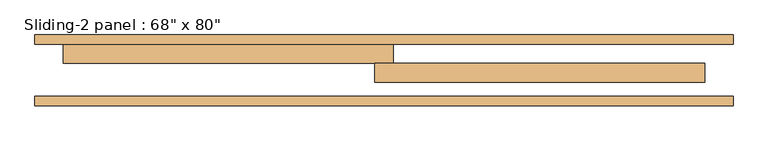
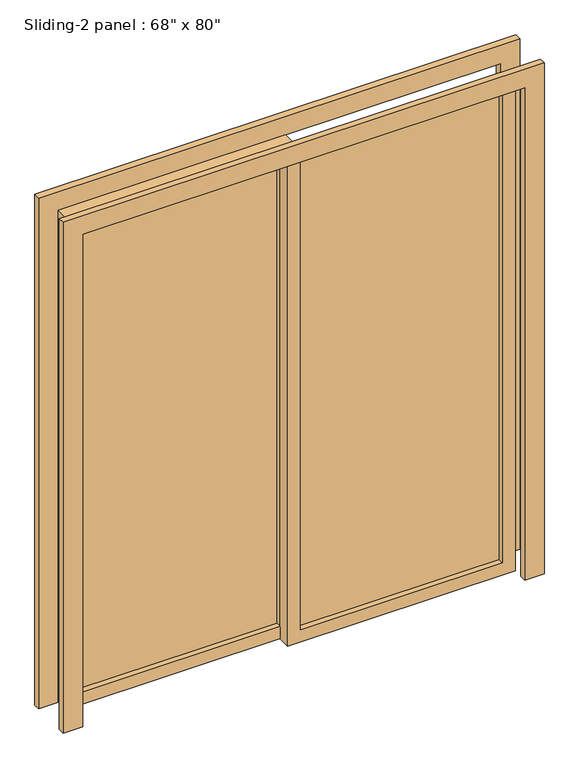
"""IFC4 building model written with IfcOpenShell, lengths in millimetres: door geometry."""

from ifc_helpers import new_model, si_unit, frame, origin, place, context, project, spatial, polyline, outline, extrude, source, transform, mapped, element, save


def door_e1f4216b(model_context):
    return source(origin(), model_context, "Body", "SweptSolid", [
        extrude(outline(polyline([(25.4, 123.825), (812.8, 123.825), (812.8, 117.475), (25.4, 117.475), (25.4, 123.825)])), frame((0.0, 0.0, 50.8), z_axis=(0.0, 0.0, 1.0), x_axis=(1.0, 0.0, 0.0)), (0.0, 0.0, 1.0), 1930.4),
        extrude(outline(polyline([(2032.0, -25.4), (0.0, -25.4), (0.0, 863.6), (2032.0, 863.6), (2032.0, -25.4)]), holes=[polyline([(1981.2, 25.4), (1981.2, 812.8), (50.8, 812.8), (50.8, 25.4), (1981.2, 25.4)])]), frame((0.0, 95.25, 0.0), z_axis=(0.0, 1.0, 0.0), x_axis=(0.0, 0.0, 1.0)), (0.0, 0.0, 1.0), 50.8),
        extrude(outline(polyline([(-812.8, 174.625), (-25.4, 174.625), (-25.4, 168.275), (-812.8, 168.275), (-812.8, 174.625)])), frame((0.0, 0.0, 50.8), z_axis=(0.0, 0.0, 1.0), x_axis=(1.0, 0.0, 0.0)), (0.0, 0.0, 1.0), 1930.4),
        extrude(outline(polyline([(2032.0, 25.4), (2032.0, -863.6), (0.0, -863.6), (0.0, 25.4), (2032.0, 25.4)]), holes=[polyline([(1981.2, -25.4), (50.8, -25.4), (50.8, -812.8), (1981.2, -812.8), (1981.2, -25.4)])]), frame((0.0, 146.05, 0.0), z_axis=(0.0, 1.0, 0.0), x_axis=(0.0, 0.0, 1.0)), (0.0, 0.0, 1.0), 50.8),
        extrude(outline(polyline([(0.0, -939.8), (0.0, -863.6), (2032.0, -863.6), (2032.0, 863.6), (0.0, 863.6), (0.0, 939.8), (2108.2, 939.8), (2108.2, -939.8), (0.0, -939.8)])), frame((0.0, 31.75, 0.0), z_axis=(0.0, 1.0, 0.0), x_axis=(0.0, 0.0, 1.0)), (0.0, 0.0, 1.0), 25.4),
        extrude(outline(polyline([(0.0, 939.8), (2108.2, 939.8), (2108.2, -939.8), (0.0, -939.8), (0.0, -863.6), (2032.0, -863.6), (2032.0, 863.6), (0.0, 863.6), (0.0, 939.8)])), frame((0.0, 196.85, 0.0), z_axis=(0.0, 1.0, 0.0), x_axis=(0.0, 0.0, 1.0)), (0.0, 0.0, 1.0), 25.4),
    ])


if __name__ == "__main__":
    model = new_model("IFC4")
    model_context = context("Model", 3, world=origin())
    ifc_project = project(units=[si_unit("LENGTHUNIT", "METRE", prefix="MILLI")], contexts=[model_context])
    site = spatial("IfcSite", under=ifc_project)
    building = spatial("IfcBuilding", under=site)
    placement = place(None, origin())
    door_shape = door_e1f4216b(model_context)
    element("IfcDoor", 1, ObjectType="Sliding-2 panel : 68\" x 80\"", at=placement, inside=building, context=model_context, shape_type="MappedRepresentation", body=[
        mapped(door_shape, transform((0.0, 0.0, 0.0), x_axis=(1.0, 0.0, 0.0), y_axis=(0.0, 1.0, 0.0), z_axis=(0.0, 0.0, 1.0))),
    ])
    save(model, "model.ifc")

# Revit data of these elements
# Type "Sliding-2 panel : 68\" x 80\""
#   Type Mark = "2"
#   Assembly Code = "C1020"
#   Thickness = 0' - 2"
#   Height = 6' - 8"
#   Rail Width = 0' - 2"
#   Stile Width = 0' - 2"
#   Trim Projection Ext = 0' - 1"
#   Trim Projection Int = 0' - 1"
#   Trim Width = 0' - 3"
#   Width = 5' - 8"
#   Function = 0
#   Door Material = Door - Panel
#   Frame Material = Metal - Aluminum
#   Wall Closure = (empty or 0)
# Element 1 (IfcDoor, "Sliding-2 panel : 68\" x 80\"")
#   Materials on its faces: "Door - Panel", "Metal - Aluminum", "Glass"
# Materials
#   "Door - Panel": class "Wood", colour RGB 149 143 132, transparency 0, Comments = "Rendering appearance not upgraded Rendering appearance not upgraded "
#   "Metal - Aluminum": class "Metal", colour RGB 244 244 244, transparency 0, Comments = "Rendering appearance not upgraded Rendering appearance not upgraded ", Description = "Aluminum"
#   "Glass": class "Glass", colour RGB 218 227 224, transparency 0.7, Comments = "Rendering appearance not upgraded Rendering appearance not upgraded ", Description = "Glass"
